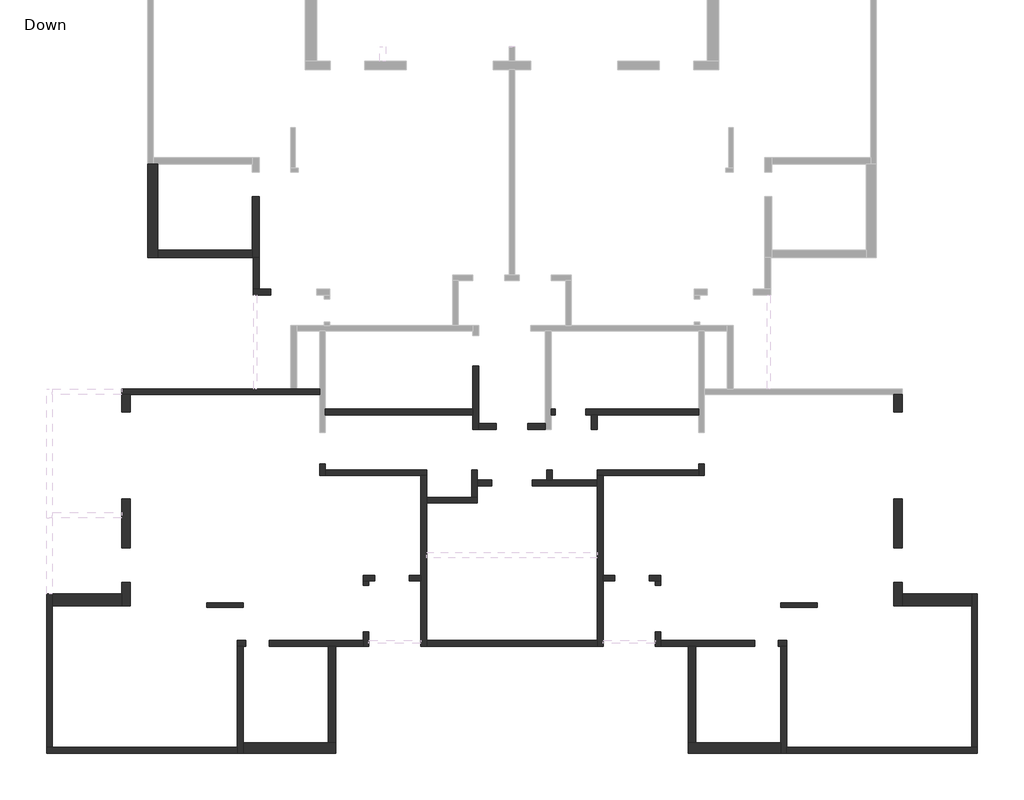
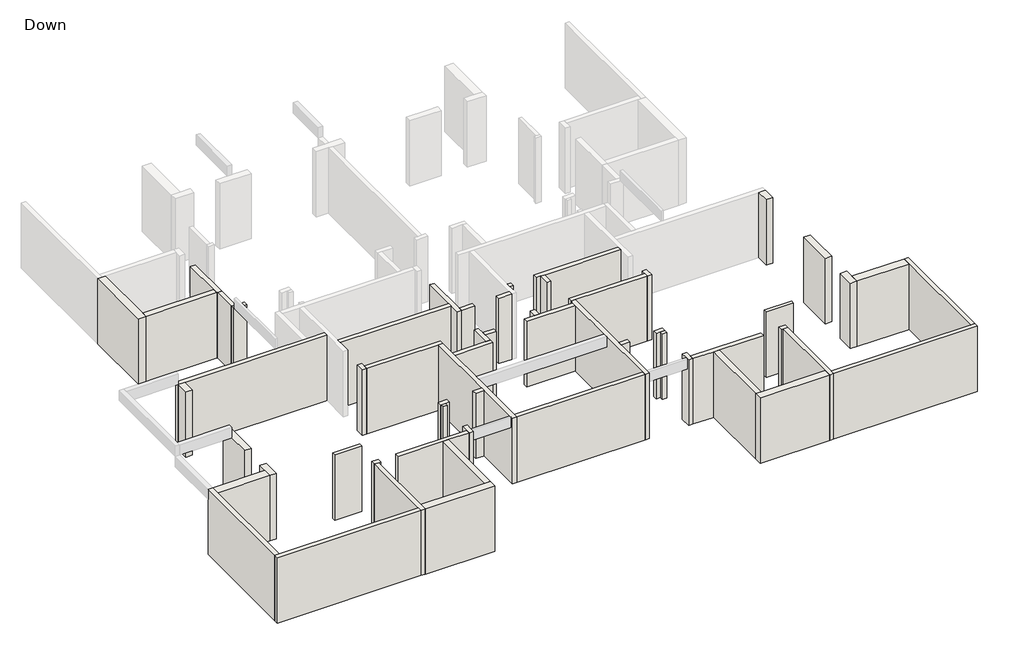
# One storey, part 1 of 2: 57 walls.
# Revit data of these elements (continued)
# Project information (continued)
#   IfcBuilding GUID = "0qmWcHnSX2jgDgeekqEEDW"
#   IfcProject GUID = "0qmWcHnSX2jgDgeekqEEDX"
#   Project Issue Date = "Issue Date"
#   Project Status = "Project Status"
#   Client Name = "לקוח"
#   Project Address = "Enter address here"
#   Project Name = "Project 028"
#   Project Number = "מספר פרויקט"
# Type "15"
#   Type IfcGUID = "1e7LVzuKbECxrDX1g1kHgD"
#   Layers, outside or top first: 15 cm "Concrete" (function 1)
# Type "20"
#   Type IfcGUID = "1qv6ynVKX7xf87anS8vNv6"
#   Layers, outside or top first: 20 cm "Concrete" (function 1)
# Type "23"
#   Type IfcGUID = "1e7LVzuKbECxrDX1g1kMy_"
#   Layers, outside or top first: 23 cm "Concrete" (function 1)
# Type "25"
#   Type IfcGUID = "1zn3TUKgbD69x5FAYjkTCE"
#   Layers, outside or top first: 25 cm "Concrete" (function 1)
# Type "30"
#   Type IfcGUID = "1qv6ynVKX7xf87anS8vNvn"
#   Layers, outside or top first: 30 cm "Concrete" (function 1)
# Type "35"
#   Type IfcGUID = "1zn3TUKgbD69x5FAYjkTCO"
#   Layers, outside or top first: 35 cm "Concrete" (function 1)
# Type "40"
#   Type IfcGUID = "1zn3TUKgbD69x5FAYjkTCY"
#   Layers, outside or top first: 40 cm "Concrete" (function 1)
# Element 1 (IfcWall, "15")
#   IfcGUID = "1e7LVzuKbECxrDX1g1kGXb"
#   Comments = ""
#   Mark = "W94"
#   SOFiSTiK_EdgeZones = "W85"
#   SOFiSTiK_AMG_Comments = ""
#   Top Offset = 0 cm
#   Base Offset = 0 cm
#   wall height = 318 cm
#   SOFiSTiK_AMG_Scheduled = yes
#   SOFiSTiK_AMG_Adjusted = yes
#   Phase Created = New Construction
#   Base Constraint = Down
#   Top Constraint = Typical Floor
#   Materials on its faces: "Concrete"
# Element 2 (IfcWall, "15")
#   IfcGUID = "3brXM_Qu1DvOaG$o2DBD1Y"
#   Comments = ""
#   Mark = "W97"
#   SOFiSTiK_EdgeZones = "W88"
#   SOFiSTiK_AMG_Comments = ""
#   Top Offset = 0 cm
#   Base Offset = 0 cm
#   wall height = 318 cm
#   SOFiSTiK_AMG_Scheduled = yes
#   SOFiSTiK_AMG_Adjusted = yes
#   Phase Created = New Construction
#   Base Constraint = Down
#   Top Constraint = Typical Floor
#   Materials on its faces: "Concrete"
# Element 3 (IfcWall, "20")
#   IfcGUID = "1e7LVzuKbECxrDX1g1kMob"
#   Comments = ""
#   Mark = "W2"
#   SOFiSTiK_EdgeZones = "W2"
#   SOFiSTiK_AMG_Comments = ""
#   Top Offset = 0 cm
#   Base Offset = 0 cm
#   wall height = 318 cm
#   SOFiSTiK_AMG_Scheduled = yes
#   SOFiSTiK_AMG_Adjusted = yes
#   Phase Created = New Construction
#   Base Constraint = Down
#   Top Constraint = Typical Floor
#   Materials on its faces: "Concrete"
# Element 4 (IfcWall, "20")
#   IfcGUID = "1e7LVzuKbECxrDX1g1kMph"
#   Comments = ""
#   Mark = "W3"
#   SOFiSTiK_EdgeZones = "W3"
#   SOFiSTiK_AMG_Comments = ""
#   Top Offset = 0 cm
#   Base Offset = 0 cm
#   wall height = 318 cm
#   SOFiSTiK_AMG_Scheduled = yes
#   SOFiSTiK_AMG_Adjusted = yes
#   Phase Created = New Construction
#   Base Constraint = Down
#   Top Constraint = Typical Floor
#   Materials on its faces: "Concrete"
# Element 5 (IfcWall, "20")
#   IfcGUID = "1e7LVzuKbECxrDX1g1kH3W"
#   Comments = ""
#   Mark = "W9"
#   SOFiSTiK_EdgeZones = "W9"
#   SOFiSTiK_AMG_Comments = ""
#   Top Offset = 0 cm
#   Base Offset = 0 cm
#   wall height = 318 cm
#   SOFiSTiK_AMG_Scheduled = yes
#   SOFiSTiK_AMG_Adjusted = yes
#   Phase Created = New Construction
#   Base Constraint = Down
#   Top Constraint = Typical Floor
#   Materials on its faces: "Concrete"
# Element 6 (IfcWall, "20")
#   IfcGUID = "1e7LVzuKbECxrDX1g1kH0x"
#   Comments = ""
#   Mark = "W10"
#   SOFiSTiK_EdgeZones = "W10"
#   SOFiSTiK_AMG_Comments = ""
#   Top Offset = 0 cm
#   Base Offset = 0 cm
#   wall height = 318 cm
#   SOFiSTiK_AMG_Scheduled = yes
#   SOFiSTiK_AMG_Adjusted = yes
#   Phase Created = New Construction
#   Base Constraint = Down
#   Top Constraint = Typical Floor
#   Materials on its faces: "Concrete"
# Element 7 (IfcWall, "20")
#   IfcGUID = "1e7LVzuKbECxrDX1g1kHV8"
#   Comments = ""
#   Mark = "W11"
#   SOFiSTiK_EdgeZones = "W11"
#   SOFiSTiK_AMG_Comments = ""
#   Top Offset = 0 cm
#   Base Offset = 0 cm
#   wall height = 318 cm
#   SOFiSTiK_AMG_Scheduled = yes
#   SOFiSTiK_AMG_Adjusted = yes
#   Phase Created = New Construction
#   Base Constraint = Down
#   Top Constraint = Typical Floor
#   Materials on its faces: "Concrete"
# Element 8 (IfcWall, "20")
#   IfcGUID = "1e7LVzuKbECxrDX1g1kHiP"
#   Comments = ""
#   Mark = "W17"
#   SOFiSTiK_EdgeZones = "W14"
#   SOFiSTiK_AMG_Comments = ""
#   Top Offset = 0 cm
#   Base Offset = 0 cm
#   wall height = 318 cm
#   SOFiSTiK_AMG_Scheduled = yes
#   SOFiSTiK_AMG_Adjusted = yes
#   Phase Created = New Construction
#   Base Constraint = Down
#   Top Constraint = Typical Floor
#   Materials on its faces: "Concrete"
# Element 9 (IfcWall, "20")
#   IfcGUID = "1e7LVzuKbECxrDX1g1kG9S"
#   Comments = ""
#   Mark = "W25"
#   SOFiSTiK_EdgeZones = "W21"
#   SOFiSTiK_AMG_Comments = ""
#   Top Offset = 0 cm
#   Base Offset = 0 cm
#   wall height = 318 cm
#   SOFiSTiK_AMG_Scheduled = yes
#   SOFiSTiK_AMG_Adjusted = yes
#   Phase Created = New Construction
#   Base Constraint = Down
#   Top Constraint = Typical Floor
#   Materials on its faces: "Concrete"
# Element 10 (IfcWall, "20")
#   IfcGUID = "1e7LVzuKbECxrDX1g1kG6f"
#   Comments = ""
#   Mark = "W26"
#   SOFiSTiK_EdgeZones = "W22"
#   SOFiSTiK_AMG_Comments = ""
#   Top Offset = 0 cm
#   Base Offset = 0 cm
#   wall height = 318 cm
#   SOFiSTiK_AMG_Scheduled = yes
#   SOFiSTiK_AMG_Adjusted = yes
#   Phase Created = New Construction
#   Base Constraint = Down
#   Top Constraint = Typical Floor
#   Materials on its faces: "Concrete"
# Element 11 (IfcWall, "20")
#   IfcGUID = "1e7LVzuKbECxrDX1g1kG2Q"
#   Comments = ""
#   Mark = "W27"
#   SOFiSTiK_EdgeZones = "W23"
#   SOFiSTiK_AMG_Comments = ""
#   Top Offset = 0 cm
#   Base Offset = 0 cm
#   wall height = 318 cm
#   SOFiSTiK_AMG_Scheduled = yes
#   SOFiSTiK_AMG_Adjusted = yes
#   Phase Created = New Construction
#   Base Constraint = Down
#   Top Constraint = Typical Floor
#   Materials on its faces: "Concrete"
# Element 12 (IfcWall, "20")
#   IfcGUID = "1e7LVzuKbECxrDX1g1kG0o"
#   Comments = ""
#   Mark = "W28"
#   SOFiSTiK_EdgeZones = "W24"
#   SOFiSTiK_AMG_Comments = ""
#   Top Offset = 0 cm
#   Base Offset = 0 cm
#   wall height = 318 cm
#   SOFiSTiK_AMG_Scheduled = yes
#   SOFiSTiK_AMG_Adjusted = yes
#   Phase Created = New Construction
#   Base Constraint = Down
#   Top Constraint = Typical Floor
#   Materials on its faces: "Concrete"
# Element 13 (IfcWall, "20")
#   IfcGUID = "1e7LVzuKbECxrDX1g1kG1f"
#   Comments = ""
#   Mark = "W29"
#   SOFiSTiK_EdgeZones = "W25"
#   SOFiSTiK_AMG_Comments = ""
#   Top Offset = 0 cm
#   Base Offset = 0 cm
#   wall height = 318 cm
#   SOFiSTiK_AMG_Scheduled = yes
#   SOFiSTiK_AMG_Adjusted = yes
#   Phase Created = New Construction
#   Base Constraint = Down
#   Top Constraint = Typical Floor
#   Materials on its faces: "Concrete"
# Element 14 (IfcWall, "20")
#   IfcGUID = "1e7LVzuKbECxrDX1g1kGUw"
#   Comments = ""
#   Mark = "W30"
#   SOFiSTiK_EdgeZones = "W26"
#   SOFiSTiK_AMG_Comments = ""
#   Top Offset = 0 cm
#   Base Offset = 0 cm
#   wall height = 318 cm
#   SOFiSTiK_AMG_Scheduled = yes
#   SOFiSTiK_AMG_Adjusted = yes
#   Phase Created = New Construction
#   Base Constraint = Down
#   Top Constraint = Typical Floor
#   Materials on its faces: "Concrete"
# Element 15 (IfcWall, "20")
#   IfcGUID = "1e7LVzuKbECxrDX1g1kGT9"
#   Comments = ""
#   Mark = "W31"
#   SOFiSTiK_EdgeZones = "W27"
#   SOFiSTiK_AMG_Comments = ""
#   Top Offset = 0 cm
#   Base Offset = 0 cm
#   wall height = 318 cm
#   SOFiSTiK_AMG_Scheduled = yes
#   SOFiSTiK_AMG_Adjusted = yes
#   Phase Created = New Construction
#   Base Constraint = Down
#   Top Constraint = Typical Floor
#   Materials on its faces: "Concrete"
# Element 16 (IfcWall, "20")
#   IfcGUID = "1e7LVzuKbECxrDX1g1kGOK"
#   Comments = ""
#   Mark = "W32"
#   SOFiSTiK_EdgeZones = "W28"
#   SOFiSTiK_AMG_Comments = ""
#   Top Offset = 0 cm
#   Base Offset = 0 cm
#   wall height = 318 cm
#   SOFiSTiK_AMG_Scheduled = yes
#   SOFiSTiK_AMG_Adjusted = yes
#   Phase Created = New Construction
#   Base Constraint = Down
#   Top Constraint = Typical Floor
#   Materials on its faces: "Concrete"
# Element 17 (IfcWall, "20")
#   IfcGUID = "1e7LVzuKbECxrDX1g1kGMI"
#   Comments = ""
#   Mark = "W33"
#   SOFiSTiK_EdgeZones = "W29"
#   SOFiSTiK_AMG_Comments = ""
#   Top Offset = 0 cm
#   Base Offset = 0 cm
#   wall height = 318 cm
#   SOFiSTiK_AMG_Scheduled = yes
#   SOFiSTiK_AMG_Adjusted = yes
#   Phase Created = New Construction
#   Base Constraint = Down
#   Top Constraint = Typical Floor
#   Materials on its faces: "Concrete"
# Element 18 (IfcWall, "20")
#   IfcGUID = "1e7LVzuKbECxrDX1g1kGK$"
#   Comments = ""
#   Mark = "W34"
#   SOFiSTiK_EdgeZones = "W30"
#   SOFiSTiK_AMG_Comments = ""
#   Top Offset = 0 cm
#   Base Offset = 0 cm
#   wall height = 318 cm
#   SOFiSTiK_AMG_Scheduled = yes
#   SOFiSTiK_AMG_Adjusted = yes
#   Phase Created = New Construction
#   Base Constraint = Down
#   Top Constraint = Typical Floor
#   Materials on its faces: "Concrete"
# Element 19 (IfcWall, "20")
#   IfcGUID = "1e7LVzuKbECxrDX1g1kGG5"
#   Comments = ""
#   Mark = "W35"
#   SOFiSTiK_EdgeZones = "W31"
#   SOFiSTiK_AMG_Comments = ""
#   Top Offset = 0 cm
#   Base Offset = 0 cm
#   wall height = 318 cm
#   SOFiSTiK_AMG_Scheduled = yes
#   SOFiSTiK_AMG_Adjusted = yes
#   Phase Created = New Construction
#   Base Constraint = Down
#   Top Constraint = Typical Floor
#   Materials on its faces: "Concrete"
# Element 20 (IfcWall, "20")
#   IfcGUID = "1e7LVzuKbECxrDX1g1kGl4"
#   Comments = ""
#   Mark = "W36"
#   SOFiSTiK_EdgeZones = "W32"
#   SOFiSTiK_AMG_Comments = ""
#   Top Offset = 0 cm
#   Base Offset = 0 cm
#   wall height = 318 cm
#   SOFiSTiK_AMG_Scheduled = yes
#   SOFiSTiK_AMG_Adjusted = yes
#   Phase Created = New Construction
#   Base Constraint = Down
#   Top Constraint = Typical Floor
#   Materials on its faces: "Concrete"
# Element 21 (IfcWall, "20")
#   IfcGUID = "3brXM_Qu1DvOaG$o2DBD0_"
#   Comments = ""
#   Mark = "W46"
#   SOFiSTiK_EdgeZones = "W41"
#   SOFiSTiK_AMG_Comments = ""
#   Top Offset = 0 cm
#   Base Offset = 0 cm
#   wall height = 318 cm
#   SOFiSTiK_AMG_Scheduled = yes
#   SOFiSTiK_AMG_Adjusted = yes
#   Phase Created = New Construction
#   Base Constraint = Down
#   Top Constraint = Typical Floor
#   Materials on its faces: "Concrete"
# Element 22 (IfcWall, "20")
#   IfcGUID = "3brXM_Qu1DvOaG$o2DBD0W"
#   Comments = ""
#   Mark = "W47"
#   SOFiSTiK_EdgeZones = "W42"
#   SOFiSTiK_AMG_Comments = ""
#   Top Offset = 0 cm
#   Base Offset = 0 cm
#   wall height = 318 cm
#   SOFiSTiK_AMG_Scheduled = yes
#   SOFiSTiK_AMG_Adjusted = yes
#   Phase Created = New Construction
#   Base Constraint = Down
#   Top Constraint = Typical Floor
#   Materials on its faces: "Concrete"
# Element 23 (IfcWall, "20")
#   IfcGUID = "3brXM_Qu1DvOaG$o2DBD0U"
#   Comments = ""
#   Mark = "W57"
#   SOFiSTiK_EdgeZones = "W49"
#   SOFiSTiK_AMG_Comments = ""
#   Top Offset = 0 cm
#   Base Offset = 0 cm
#   wall height = 318 cm
#   SOFiSTiK_AMG_Scheduled = yes
#   SOFiSTiK_AMG_Adjusted = yes
#   Phase Created = New Construction
#   Base Constraint = Down
#   Top Constraint = Typical Floor
#   Materials on its faces: "Concrete"
# Element 24 (IfcWall, "20")
#   IfcGUID = "3brXM_Qu1DvOaG$o2DBD00"
#   Comments = ""
#   Mark = "W58"
#   SOFiSTiK_EdgeZones = "W50"
#   SOFiSTiK_AMG_Comments = ""
#   Top Offset = 0 cm
#   Base Offset = 0 cm
#   wall height = 318 cm
#   SOFiSTiK_AMG_Scheduled = yes
#   SOFiSTiK_AMG_Adjusted = yes
#   Phase Created = New Construction
#   Base Constraint = Down
#   Top Constraint = Typical Floor
#   Materials on its faces: "Concrete"
# Element 25 (IfcWall, "20")
#   IfcGUID = "3brXM_Qu1DvOaG$o2DBD02"
#   Comments = ""
#   Mark = "W59"
#   SOFiSTiK_EdgeZones = "W51"
#   SOFiSTiK_AMG_Comments = ""
#   Top Offset = 0 cm
#   Base Offset = 0 cm
#   wall height = 318 cm
#   SOFiSTiK_AMG_Scheduled = yes
#   SOFiSTiK_AMG_Adjusted = yes
#   Phase Created = New Construction
#   Base Constraint = Down
#   Top Constraint = Typical Floor
#   Materials on its faces: "Concrete"
# Element 26 (IfcWall, "20")
#   IfcGUID = "3brXM_Qu1DvOaG$o2DBD04"
#   Comments = ""
#   Mark = "W60"
#   SOFiSTiK_EdgeZones = "W52"
#   SOFiSTiK_AMG_Comments = ""
#   Top Offset = 0 cm
#   Base Offset = 0 cm
#   wall height = 318 cm
#   SOFiSTiK_AMG_Scheduled = yes
#   SOFiSTiK_AMG_Adjusted = yes
#   Phase Created = New Construction
#   Base Constraint = Down
#   Top Constraint = Typical Floor
#   Materials on its faces: "Concrete"
# Element 27 (IfcWall, "20")
#   IfcGUID = "3brXM_Qu1DvOaG$o2DBD06"
#   Comments = ""
#   Mark = "W61"
#   SOFiSTiK_EdgeZones = "W53"
#   SOFiSTiK_AMG_Comments = ""
#   Top Offset = 0 cm
#   Base Offset = 0 cm
#   wall height = 318 cm
#   SOFiSTiK_AMG_Scheduled = yes
#   SOFiSTiK_AMG_Adjusted = yes
#   Phase Created = New Construction
#   Base Constraint = Down
#   Top Constraint = Typical Floor
#   Materials on its faces: "Concrete"
# Element 28 (IfcWall, "20")
#   IfcGUID = "3brXM_Qu1DvOaG$o2DBD08"
#   Comments = ""
#   Mark = "W62"
#   SOFiSTiK_EdgeZones = "W54"
#   SOFiSTiK_AMG_Comments = ""
#   Top Offset = 0 cm
#   Base Offset = 0 cm
#   wall height = 318 cm
#   SOFiSTiK_AMG_Scheduled = yes
#   SOFiSTiK_AMG_Adjusted = yes
#   Phase Created = New Construction
#   Base Constraint = Down
#   Top Constraint = Typical Floor
#   Materials on its faces: "Concrete"
# Element 29 (IfcWall, "20")
#   IfcGUID = "3brXM_Qu1DvOaG$o2DBD0A"
#   Comments = ""
#   Mark = "W63"
#   SOFiSTiK_EdgeZones = "W55"
#   SOFiSTiK_AMG_Comments = ""
#   Top Offset = 0 cm
#   Base Offset = 0 cm
#   wall height = 318 cm
#   SOFiSTiK_AMG_Scheduled = yes
#   SOFiSTiK_AMG_Adjusted = yes
#   Phase Created = New Construction
#   Base Constraint = Down
#   Top Constraint = Typical Floor
#   Materials on its faces: "Concrete"
# Element 30 (IfcWall, "20")
#   IfcGUID = "3brXM_Qu1DvOaG$o2DBD0C"
#   Comments = ""
#   Mark = "W64"
#   SOFiSTiK_EdgeZones = "W56"
#   SOFiSTiK_AMG_Comments = ""
#   Top Offset = 0 cm
#   Base Offset = 0 cm
#   wall height = 318 cm
#   SOFiSTiK_AMG_Scheduled = yes
#   SOFiSTiK_AMG_Adjusted = yes
#   Phase Created = New Construction
#   Base Constraint = Down
#   Top Constraint = Typical Floor
#   Materials on its faces: "Concrete"
# Element 31 (IfcWall, "20")
#   IfcGUID = "3brXM_Qu1DvOaG$o2DBD0E"
#   Comments = ""
#   Mark = "W65"
#   SOFiSTiK_EdgeZones = "W57"
#   SOFiSTiK_AMG_Comments = ""
#   Top Offset = 0 cm
#   Base Offset = 0 cm
#   wall height = 318 cm
#   SOFiSTiK_AMG_Scheduled = yes
#   SOFiSTiK_AMG_Adjusted = yes
#   Phase Created = New Construction
#   Base Constraint = Down
#   Top Constraint = Typical Floor
#   Materials on its faces: "Concrete"
# Element 32 (IfcWall, "20")
#   IfcGUID = "3brXM_Qu1DvOaG$o2DBD1m"
#   Comments = ""
#   Mark = "W66"
#   SOFiSTiK_EdgeZones = "W58"
#   SOFiSTiK_AMG_Comments = ""
#   Top Offset = 0 cm
#   Base Offset = 0 cm
#   wall height = 318 cm
#   SOFiSTiK_AMG_Scheduled = yes
#   SOFiSTiK_AMG_Adjusted = yes
#   Phase Created = New Construction
#   Base Constraint = Down
#   Top Constraint = Typical Floor
#   Materials on its faces: "Concrete"
# Element 33 (IfcWall, "20")
#   IfcGUID = "3brXM_Qu1DvOaG$o2DBD1o"
#   Comments = ""
#   Mark = "W67"
#   SOFiSTiK_EdgeZones = "W59"
#   SOFiSTiK_AMG_Comments = ""
#   Top Offset = 0 cm
#   Base Offset = 0 cm
#   wall height = 318 cm
#   SOFiSTiK_AMG_Scheduled = yes
#   SOFiSTiK_AMG_Adjusted = yes
#   Phase Created = New Construction
#   Base Constraint = Down
#   Top Constraint = Typical Floor
#   Materials on its faces: "Concrete"
# Element 34 (IfcWall, "20")
#   IfcGUID = "3brXM_Qu1DvOaG$o2DBD1q"
#   Comments = ""
#   Mark = "W68"
#   SOFiSTiK_EdgeZones = "W60"
#   SOFiSTiK_AMG_Comments = ""
#   Top Offset = 0 cm
#   Base Offset = 0 cm
#   wall height = 318 cm
#   SOFiSTiK_AMG_Scheduled = yes
#   SOFiSTiK_AMG_Adjusted = yes
#   Phase Created = New Construction
#   Base Constraint = Down
#   Top Constraint = Typical Floor
#   Materials on its faces: "Concrete"
# Element 35 (IfcWall, "20")
#   IfcGUID = "3brXM_Qu1DvOaG$o2DBDEp"
#   Comments = ""
#   Mark = "W69"
#   SOFiSTiK_EdgeZones = "W61"
#   SOFiSTiK_AMG_Comments = ""
#   Top Offset = 0 cm
#   Base Offset = 0 cm
#   wall height = 318 cm
#   SOFiSTiK_AMG_Scheduled = yes
#   SOFiSTiK_AMG_Adjusted = yes
#   Phase Created = New Construction
#   Base Constraint = Down
#   Top Constraint = Typical Floor
#   Materials on its faces: "Concrete"
# Element 36 (IfcWall, "20")
#   IfcGUID = "3brXM_Qu1DvOaG$o2DB2qe"
#   Comments = ""
#   Mark = "W71"
#   SOFiSTiK_EdgeZones = "W62"
#   SOFiSTiK_AMG_Comments = "Too Short /"
#   Top Offset = 0 cm
#   Base Offset = 0 cm
#   wall height = 318 cm
#   SOFiSTiK_AMG_Scheduled = yes
#   SOFiSTiK_AMG_Adjusted = yes
#   Phase Created = New Construction
#   Base Constraint = Down
#   Top Constraint = Typical Floor
#   Materials on its faces: "Concrete"
# Element 37 (IfcWall, "20")
#   IfcGUID = "3brXM_Qu1DvOaG$o2DB2tj"
#   Comments = ""
#   Mark = "W72"
#   SOFiSTiK_EdgeZones = "W63"
#   SOFiSTiK_AMG_Comments = ""
#   Top Offset = 0 cm
#   Base Offset = 0 cm
#   wall height = 318 cm
#   SOFiSTiK_AMG_Scheduled = yes
#   SOFiSTiK_AMG_Adjusted = yes
#   Phase Created = New Construction
#   Base Constraint = Down
#   Top Constraint = Typical Floor
#   Materials on its faces: "Concrete"
# Element 38 (IfcWall, "20")
#   IfcGUID = "3brXM_Qu1DvOaG$o2DB2we"
#   Comments = ""
#   Mark = "W73"
#   SOFiSTiK_EdgeZones = "W64"
#   SOFiSTiK_AMG_Comments = ""
#   Top Offset = 0 cm
#   Base Offset = 0 cm
#   wall height = 318 cm
#   SOFiSTiK_AMG_Scheduled = yes
#   SOFiSTiK_AMG_Adjusted = yes
#   Phase Created = New Construction
#   Base Constraint = Down
#   Top Constraint = Typical Floor
#   Materials on its faces: "Concrete"
# Element 39 (IfcWall, "20")
#   IfcGUID = "3brXM_Qu1DvOaG$o2DB2xT"
#   Comments = ""
#   Mark = "W74"
#   SOFiSTiK_EdgeZones = "W65"
#   SOFiSTiK_AMG_Comments = ""
#   Top Offset = 0 cm
#   Base Offset = 0 cm
#   wall height = 318 cm
#   SOFiSTiK_AMG_Scheduled = yes
#   SOFiSTiK_AMG_Adjusted = yes
#   Phase Created = New Construction
#   Base Constraint = Down
#   Top Constraint = Typical Floor
#   Materials on its faces: "Concrete"
# Element 40 (IfcWall, "20")
#   IfcGUID = "3brXM_Qu1DvOaG$o2DB2zm"
#   Comments = ""
#   Mark = "W75"
#   SOFiSTiK_EdgeZones = "W66"
#   SOFiSTiK_AMG_Comments = ""
#   Top Offset = 0 cm
#   Base Offset = 0 cm
#   wall height = 318 cm
#   SOFiSTiK_AMG_Scheduled = yes
#   SOFiSTiK_AMG_Adjusted = yes
#   Phase Created = New Construction
#   Base Constraint = Down
#   Top Constraint = Typical Floor
#   Materials on its faces: "Concrete"
# Element 41 (IfcWall, "20")
#   IfcGUID = "3brXM_Qu1DvOaG$o2DB2Ys"
#   Comments = ""
#   Mark = "W76"
#   SOFiSTiK_EdgeZones = "W67"
#   SOFiSTiK_AMG_Comments = ""
#   Top Offset = 0 cm
#   Base Offset = 0 cm
#   wall height = 318 cm
#   SOFiSTiK_AMG_Scheduled = yes
#   SOFiSTiK_AMG_Adjusted = yes
#   Phase Created = New Construction
#   Base Constraint = Down
#   Top Constraint = Typical Floor
#   Materials on its faces: "Concrete"
# Element 42 (IfcWall, "20")
#   IfcGUID = "3brXM_Qu1DvOaG$o2DB2Zh"
#   Comments = ""
#   Mark = "W77"
#   SOFiSTiK_EdgeZones = "W68"
#   SOFiSTiK_AMG_Comments = ""
#   Top Offset = 0 cm
#   Base Offset = 0 cm
#   wall height = 318 cm
#   SOFiSTiK_AMG_Scheduled = yes
#   SOFiSTiK_AMG_Adjusted = yes
#   Phase Created = New Construction
#   Base Constraint = Down
#   Top Constraint = Typical Floor
#   Materials on its faces: "Concrete"
# Element 43 (IfcWall, "23")
#   IfcGUID = "1e7LVzuKbECxrDX1g1kMyS"
#   Comments = ""
#   Mark = "W80"
#   SOFiSTiK_EdgeZones = "W71"
#   SOFiSTiK_AMG_Comments = ""
#   Top Offset = 0 cm
#   Base Offset = 0 cm
#   wall height = 318 cm
#   SOFiSTiK_AMG_Scheduled = yes
#   SOFiSTiK_AMG_Adjusted = yes
#   Phase Created = New Construction
#   Base Constraint = Down
#   Top Constraint = Typical Floor
#   Materials on its faces: "Concrete"
# Element 44 (IfcWall, "25")
#   IfcGUID = "1e7LVzuKbECxrDX1g1kMqG"
#   Comments = ""
#   Mark = "W88"
#   SOFiSTiK_EdgeZones = "W79"
#   SOFiSTiK_AMG_Comments = ""
#   Top Offset = 0 cm
#   Base Offset = 0 cm
#   wall height = 318 cm
#   SOFiSTiK_AMG_Scheduled = yes
#   SOFiSTiK_AMG_Adjusted = yes
#   Phase Created = New Construction
#   Base Constraint = Down
#   Top Constraint = Typical Floor
#   Materials on its faces: "Concrete"
# Element 45 (IfcWall, "25")
#   IfcGUID = "1e7LVzuKbECxrDX1g1kGWB"
#   Comments = ""
#   Mark = "W89"
#   SOFiSTiK_EdgeZones = "W80"
#   SOFiSTiK_AMG_Comments = ""
#   Top Offset = 0 cm
#   Base Offset = 0 cm
#   wall height = 318 cm
#   SOFiSTiK_AMG_Scheduled = yes
#   SOFiSTiK_AMG_Adjusted = yes
#   Phase Created = New Construction
#   Base Constraint = Down
#   Top Constraint = Typical Floor
#   Materials on its faces: "Concrete"
# Element 46 (IfcWall, "25")
#   IfcGUID = "3brXM_Qu1DvOaG$o2DBD1W"
#   Comments = ""
#   Mark = "W91"
#   SOFiSTiK_EdgeZones = "W82"
#   SOFiSTiK_AMG_Comments = ""
#   Top Offset = 0 cm
#   Base Offset = 0 cm
#   wall height = 318 cm
#   SOFiSTiK_AMG_Scheduled = yes
#   SOFiSTiK_AMG_Adjusted = yes
#   Phase Created = New Construction
#   Base Constraint = Down
#   Top Constraint = Typical Floor
#   Materials on its faces: "Concrete"
# Element 47 (IfcWall, "30")
#   IfcGUID = "1e7LVzuKbECxrDX1g1kGhA"
#   Comments = ""
#   Mark = "W105"
#   SOFiSTiK_EdgeZones = "W96"
#   SOFiSTiK_AMG_Comments = ""
#   Top Offset = 0 cm
#   Base Offset = 0 cm
#   wall height = 318 cm
#   SOFiSTiK_AMG_Scheduled = yes
#   SOFiSTiK_AMG_Adjusted = yes
#   Phase Created = New Construction
#   Base Constraint = Down
#   Top Constraint = Typical Floor
#   Materials on its faces: "Concrete"
# Element 48 (IfcWall, "30")
#   IfcGUID = "1e7LVzuKbECxrDX1g1kGeg"
#   Comments = ""
#   Mark = "W106"
#   SOFiSTiK_EdgeZones = "W97"
#   SOFiSTiK_AMG_Comments = ""
#   Top Offset = 0 cm
#   Base Offset = 0 cm
#   wall height = 318 cm
#   SOFiSTiK_AMG_Scheduled = yes
#   SOFiSTiK_AMG_Adjusted = yes
#   Phase Created = New Construction
#   Base Constraint = Down
#   Top Constraint = Typical Floor
#   Materials on its faces: "Concrete"
# Element 49 (IfcWall, "30")
#   IfcGUID = "1e7LVzuKbECxrDX1g1kGcC"
#   Comments = ""
#   Mark = "W107"
#   SOFiSTiK_EdgeZones = "W98"
#   SOFiSTiK_AMG_Comments = ""
#   Top Offset = 0 cm
#   Base Offset = 0 cm
#   wall height = 318 cm
#   SOFiSTiK_AMG_Scheduled = yes
#   SOFiSTiK_AMG_Adjusted = yes
#   Phase Created = New Construction
#   Base Constraint = Down
#   Top Constraint = Typical Floor
#   Materials on its faces: "Concrete"
# Element 50 (IfcWall, "30")
#   IfcGUID = "3brXM_Qu1DvOaG$o2DBD1u"
#   Comments = ""
#   Mark = "W110"
#   SOFiSTiK_EdgeZones = "W101"
#   SOFiSTiK_AMG_Comments = ""
#   Top Offset = 0 cm
#   Base Offset = 0 cm
#   wall height = 318 cm
#   SOFiSTiK_AMG_Scheduled = yes
#   SOFiSTiK_AMG_Adjusted = yes
#   Phase Created = New Construction
#   Base Constraint = Down
#   Top Constraint = Typical Floor
#   Materials on its faces: "Concrete"
# Element 51 (IfcWall, "30")
#   IfcGUID = "3brXM_Qu1DvOaG$o2DBD1w"
#   Comments = ""
#   Mark = "W111"
#   SOFiSTiK_EdgeZones = "W102"
#   SOFiSTiK_AMG_Comments = ""
#   Top Offset = 0 cm
#   Base Offset = 0 cm
#   wall height = 318 cm
#   SOFiSTiK_AMG_Scheduled = yes
#   SOFiSTiK_AMG_Adjusted = yes
#   Phase Created = New Construction
#   Base Constraint = Down
#   Top Constraint = Typical Floor
#   Materials on its faces: "Concrete"
# Element 52 (IfcWall, "30")
#   IfcGUID = "3brXM_Qu1DvOaG$o2DBD1y"
#   Comments = ""
#   Mark = "W112"
#   SOFiSTiK_EdgeZones = "W103"
#   SOFiSTiK_AMG_Comments = ""
#   Top Offset = 0 cm
#   Base Offset = 0 cm
#   wall height = 318 cm
#   SOFiSTiK_AMG_Scheduled = yes
#   SOFiSTiK_AMG_Adjusted = yes
#   Phase Created = New Construction
#   Base Constraint = Down
#   Top Constraint = Typical Floor
#   Materials on its faces: "Concrete"
# Element 53 (IfcWall, "35")
#   IfcGUID = "1e7LVzuKbECxrDX1g1kMur"
#   Comments = ""
#   Mark = "W84"
#   SOFiSTiK_EdgeZones = "W75"
#   SOFiSTiK_AMG_Comments = ""
#   Top Offset = 0 cm
#   Base Offset = 0 cm
#   wall height = 318 cm
#   SOFiSTiK_AMG_Scheduled = yes
#   SOFiSTiK_AMG_Adjusted = yes
#   Phase Created = New Construction
#   Base Constraint = Down
#   Top Constraint = Typical Floor
#   Materials on its faces: "Concrete"
# Element 54 (IfcWall, "35")
#   IfcGUID = "1e7LVzuKbECxrDX1g1kGb5"
#   Comments = ""
#   Mark = "W85"
#   SOFiSTiK_EdgeZones = "W76"
#   SOFiSTiK_AMG_Comments = ""
#   Top Offset = 0 cm
#   Base Offset = 0 cm
#   wall height = 318 cm
#   SOFiSTiK_AMG_Scheduled = yes
#   SOFiSTiK_AMG_Adjusted = yes
#   Phase Created = New Construction
#   Base Constraint = Down
#   Top Constraint = Typical Floor
#   Materials on its faces: "Concrete"
# Element 55 (IfcWall, "35")
#   IfcGUID = "3brXM_Qu1DvOaG$o2DBD1_"
#   Comments = ""
#   Mark = "W87"
#   SOFiSTiK_EdgeZones = "W78"
#   SOFiSTiK_AMG_Comments = ""
#   Top Offset = 0 cm
#   Base Offset = 0 cm
#   wall height = 318 cm
#   SOFiSTiK_AMG_Scheduled = yes
#   SOFiSTiK_AMG_Adjusted = yes
#   Phase Created = New Construction
#   Base Constraint = Down
#   Top Constraint = Typical Floor
#   Materials on its faces: "Concrete"
# Element 56 (IfcWall, "40")
#   IfcGUID = "1e7LVzuKbECxrDX1g1kGjw"
#   Comments = ""
#   Mark = "W99"
#   SOFiSTiK_EdgeZones = "W90"
#   SOFiSTiK_AMG_Comments = ""
#   Top Offset = 0 cm
#   Base Offset = 0 cm
#   wall height = 318 cm
#   SOFiSTiK_AMG_Scheduled = yes
#   SOFiSTiK_AMG_Adjusted = yes
#   Phase Created = New Construction
#   Base Constraint = Down
#   Top Constraint = Typical Floor
#   Materials on its faces: "Concrete"
# Element 57 (IfcWall, "40")
#   IfcGUID = "3brXM_Qu1DvOaG$o2DBD1s"
#   Comments = ""
#   Mark = "W101"
#   SOFiSTiK_EdgeZones = "W92"
#   SOFiSTiK_AMG_Comments = ""
#   Top Offset = 0 cm
#   Base Offset = 0 cm
#   wall height = 318 cm
#   SOFiSTiK_AMG_Scheduled = yes
#   SOFiSTiK_AMG_Adjusted = yes
#   Phase Created = New Construction
#   Base Constraint = Down
#   Top Constraint = Typical Floor
#   Materials on its faces: "Concrete"
# Materials
#   "Concrete": class "Concrete", colour RGB 192 192 192, transparency 0, Keynote = "01000", Description = "Cast-in-place concrete", Cost = 0
